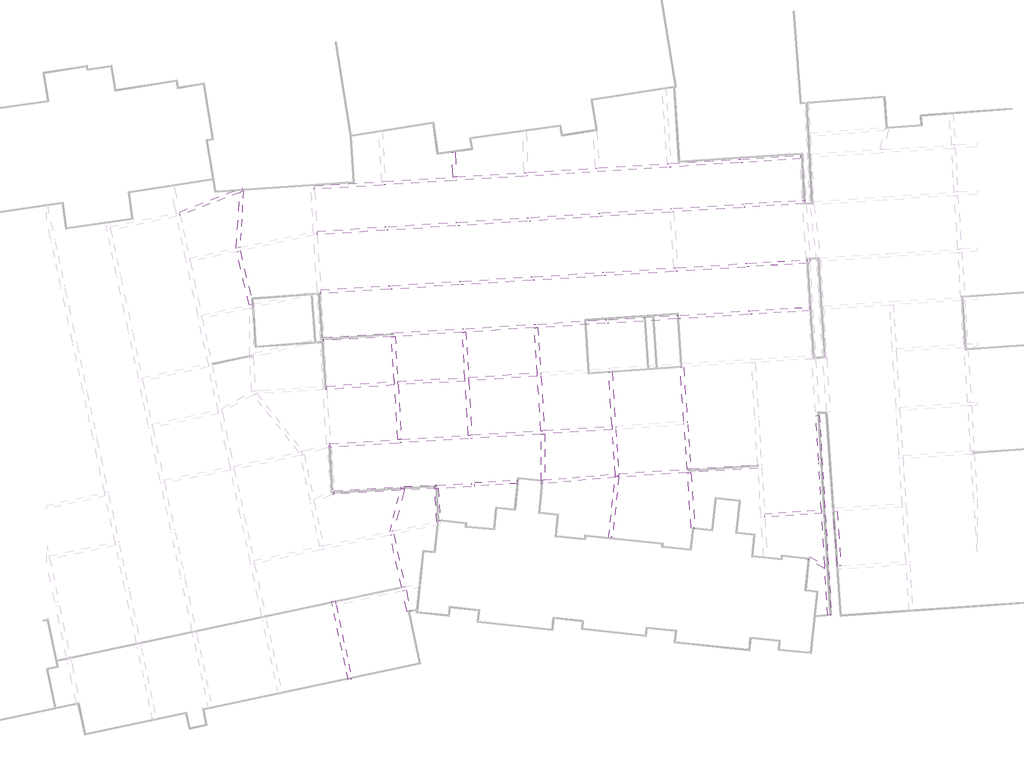
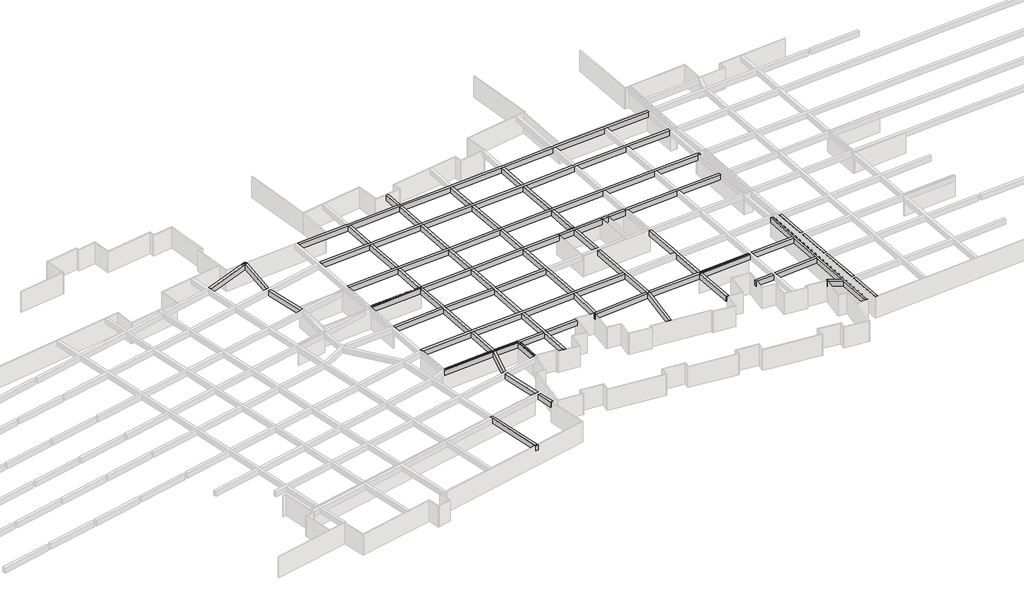
# One storey, part 11 of 14: 35 beams.
"""IFC4 building model written with IfcOpenShell, lengths in millimetres."""

import ifcopenshell
import ifcopenshell.guid

model = None  # the IFC model being written
_history = None  # IfcOwnerHistory: only IFC2X3 demands one
_inside = {}  # id of a spatial element -> (the spatial element, [elements in it])
_under = {}  # id of a project, library or spatial element -> (it, [spatial elements below it])
_declared = {}  # id of a project -> (the project, [libraries it declares])
_typed = {}  # id of a type object -> (the type object, [elements of that type])
_made_of = {}  # id of a material, layer set ... -> (it, [elements and type objects made of it])


def new_model(schema):
    """Start an empty IFC model of exactly this schema.

    Asked for "IFC4X3", IfcOpenShell would pick the latest addendum, in which some entities
    have other attributes; the version numbers below select the first issue.
    IFC2X3 requires an IfcOwnerHistory on every rooted entity: one is made here for all.
    """
    global model, _history
    if schema == "IFC4X3":
        model = ifcopenshell.file(schema_version=(4, 3, 0, 0))
    else:
        model = ifcopenshell.file(schema=schema)
    _inside.clear()
    _under.clear()
    _declared.clear()
    _typed.clear()
    _made_of.clear()
    _history = None
    if model.schema == "IFC2X3":
        org = make("IfcOrganization", Name="unknown")
        user = make(
            "IfcPersonAndOrganization",
            ThePerson=make("IfcPerson", FamilyName="unknown"),
            TheOrganization=org,
        )
        app = make(
            "IfcApplication",
            ApplicationDeveloper=org,
            Version="unknown",
            ApplicationFullName="unknown",
            ApplicationIdentifier="unknown",
        )
        _history = make(
            "IfcOwnerHistory",
            OwningUser=user,
            OwningApplication=app,
            ChangeAction="ADDED",
            CreationDate=0,
        )
    return model


def make(cls, **values):
    """One entity of the class cls with the attributes given. An attribute that is None is left unset."""
    return model.create_entity(
        cls, **{name: value for name, value in values.items() if value is not None}
    )


def rooted(cls, **values):
    """An entity with a GlobalId (a new one), such as an element, a storey or a relation."""
    return make(cls, GlobalId=ifcopenshell.guid.new(), OwnerHistory=_history, **values)


def si_unit(unit_type, name, prefix=None):
    """IfcSIUnit, for example si_unit("LENGTHUNIT", "METRE", prefix="MILLI")."""
    return make("IfcSIUnit", UnitType=unit_type, Prefix=prefix, Name=name)


def assignment(units):
    """IfcUnitAssignment: the units of a project."""
    return None if units is None else make("IfcUnitAssignment", Units=units)


def point(xyz):
    """IfcCartesianPoint."""
    return None if xyz is None else make("IfcCartesianPoint", Coordinates=xyz)


def direction(xyz):
    """IfcDirection."""
    return None if xyz is None else make("IfcDirection", DirectionRatios=xyz)


def frame(location, z_axis=None, x_axis=None):
    """IfcAxis2Placement3D, a coordinate frame: its origin and axes. An axis left out is left unset."""
    return make(
        "IfcAxis2Placement3D",
        Location=point(location),
        Axis=direction(z_axis),
        RefDirection=direction(x_axis),
    )


def origin():
    """The frame at (0, 0, 0) with its axes left unset."""
    return frame((0.0, 0.0, 0.0))


def place(relative_to, where):
    """IfcLocalPlacement: puts the frame where relative to a parent placement (None: the world)."""
    return make(
        "IfcLocalPlacement", PlacementRelTo=relative_to, RelativePlacement=where
    )


def context(
    kind, dimensions, precision=None, world=None, true_north=None, identifier=None
):
    """IfcGeometricRepresentationContext, for example the 3D "Model" context."""
    return make(
        "IfcGeometricRepresentationContext",
        ContextIdentifier=identifier,
        ContextType=kind,
        CoordinateSpaceDimension=dimensions,
        Precision=precision,
        WorldCoordinateSystem=world,
        TrueNorth=true_north,
    )


def project(units=None, contexts=None):
    """IfcProject with its units and contexts."""
    return rooted(
        "IfcProject",
        Name="project",
        RepresentationContexts=contexts,
        UnitsInContext=assignment(units),
    )


def spatial(cls, under=None, at=None, **own):
    """A site, building, storey or space (cls), placed at a placement, below another one or the project."""
    s = rooted(cls, ObjectPlacement=at, **own)
    if under is not None:
        _under.setdefault(under.id(), (under, []))[1].append(s)
    return s


def polyline(points):
    """IfcPolyline through the points."""
    return make("IfcPolyline", Points=[point(p) for p in points])


def outline(outer, holes=None, kind="AREA"):
    """IfcArbitraryClosedProfileDef: a profile drawn as a closed curve; with holes, ...WithVoids."""
    if holes is None:
        return make("IfcArbitraryClosedProfileDef", ProfileType=kind, OuterCurve=outer)
    return make(
        "IfcArbitraryProfileDefWithVoids",
        ProfileType=kind,
        OuterCurve=outer,
        InnerCurves=holes,
    )


def extrude(swept, where, along, depth):
    """IfcExtrudedAreaSolid: the profile swept, set in the frame where, extruded along a direction by depth."""
    return make(
        "IfcExtrudedAreaSolid",
        SweptArea=swept,
        Position=where,
        ExtrudedDirection=direction(along),
        Depth=depth,
    )


def faces_of(points, faces, orient=None, outer=None):
    """IfcFace entities. A face is a list of loops; a loop is a list of indices into points, from 0.

    orient and outer hold one flag for each loop. By default every Orientation is true, the
    first loop of a face is its IfcFaceOuterBound and the others are IfcFaceBound.
    """
    made = []
    for i, loops in enumerate(faces):
        bounds = []
        for j, loop in enumerate(loops):
            is_outer = j == 0 if outer is None else outer[i][j]
            bounds.append(
                make(
                    "IfcFaceOuterBound" if is_outer else "IfcFaceBound",
                    Bound=make("IfcPolyLoop", Polygon=[points[k] for k in loop]),
                    Orientation=True if orient is None else orient[i][j],
                )
            )
        made.append(make("IfcFace", Bounds=bounds))
    return made


def faceted_brep(points, faces, orient=None, outer=None, voids=None):
    """IfcFacetedBrep: a solid bounded by flat faces; with voids (closed shells), ...WithVoids."""
    shared = [point(p) for p in points]
    hull = make("IfcClosedShell", CfsFaces=faces_of(shared, faces, orient, outer))
    if voids is None:
        return make("IfcFacetedBrep", Outer=hull)
    return make(
        "IfcFacetedBrepWithVoids",
        Outer=hull,
        Voids=[
            make(cls, CfsFaces=faces_of(shared, fs, o, b)) for cls, fs, o, b in voids
        ],
    )


def shape(context_of_items, identifier, shape_type, items):
    """IfcShapeRepresentation: the items that make up one representation, for example the "Body"."""
    return make(
        "IfcShapeRepresentation",
        ContextOfItems=context_of_items,
        RepresentationIdentifier=identifier,
        RepresentationType=shape_type,
        Items=items,
    )


def made_of(thing, what):
    """Note that an element or type object is made of a material, layer set ...; save() writes the relation."""
    if what is not None:
        _made_of.setdefault(what.id(), (what, []))[1].append(thing)
    return thing


def element(
    cls,
    number,
    at=None,
    inside=None,
    cuts=None,
    type_object=None,
    material=None,
    context=None,
    identifier="Body",
    shape_type=None,
    held_by="IfcProductDefinitionShape",
    body=None,
    shapes=None,
    **own,
):
    """One element of the class cls, such as IfcWall. Its Tag is "e" and its number.

    at: its placement. inside: the storey or other place that contains it. cuts: it is an
    opening in that element (IfcRelVoidsElement). A single representation is given by context,
    identifier, shape_type and body (its items); several are given by shapes. held_by: the class
    of the entity that holds the representations. save() writes the other relations.
    """
    e = rooted(cls, Tag="e%d" % number, ObjectPlacement=at, **own)
    if body is not None:
        shapes = [shape(context, identifier, shape_type, body)]
    if shapes is not None:
        e.Representation = make(held_by, Representations=shapes)
    if inside is not None:
        _inside.setdefault(inside.id(), (inside, []))[1].append(e)
    if cuts is not None:
        rooted(
            "IfcRelVoidsElement", RelatingBuildingElement=cuts, RelatedOpeningElement=e
        )
    if type_object is not None:
        _typed.setdefault(type_object.id(), (type_object, []))[1].append(e)
    return made_of(e, material)


def aggregate(whole, parts):
    """IfcRelAggregates: a whole, such as a stair, and the parts it consists of."""
    return rooted("IfcRelAggregates", RelatingObject=whole, RelatedObjects=parts)


def save(model, path):
    """Write the relations noted so far, then the file.

    IfcRelAggregates (storeys below a building ...), IfcRelContainedInSpatialStructure (elements
    in a storey), IfcRelDefinesByType, IfcRelAssociatesMaterial and IfcRelDeclares: one each for
    every whole, place, type object, material and project.
    """
    for whole, parts in _under.values():
        aggregate(whole, parts)
    for where, things in _inside.values():
        rooted(
            "IfcRelContainedInSpatialStructure",
            RelatedElements=things,
            RelatingStructure=where,
        )
    for kind, things in _typed.values():
        rooted("IfcRelDefinesByType", RelatedObjects=things, RelatingType=kind)
    for what, things in _made_of.values():
        rooted("IfcRelAssociatesMaterial", RelatedObjects=things, RelatingMaterial=what)
    for by, libraries in _declared.values():
        rooted("IfcRelDeclares", RelatingContext=by, RelatedDefinitions=libraries)
    model.write(path)


model = new_model("IFC4")

# Units and contexts
model_context = context("Model", 3, world=origin())
ifc_project = project(units=[si_unit("LENGTHUNIT", "METRE", prefix="MILLI")], contexts=[model_context])

# Site, building, storey
site = spatial("IfcSite", under=ifc_project)
building = spatial("IfcBuilding", under=site)
storey = spatial("IfcBuildingStorey", under=building, Name="户型图", Elevation=0.0)

# Beams
placement = place(None, origin())
element("IfcBeam", 1, ObjectType="混凝土 - 矩形梁 : KL_beam", at=placement, inside=storey, context=model_context, shape_type="SweptSolid", body=[
    extrude(outline(polyline([(-202914.7402599, -137877.8870148), (-202523.4216199, -137794.7096702), (-201143.0968024, -143773.5533155), (-201534.4154425, -143856.7306602), (-202914.7402599, -137877.8870148)])), frame((0.0, 0.0, 2500.0), z_axis=(0.0, 0.0, 1.0), x_axis=(1.0, 0.0, 0.0)), (0.0, 0.0, 1.0), 800.0),
])
element("IfcBeam", 2, ObjectType="混凝土 - 矩形梁 : KL_beam", at=placement, inside=storey, context=model_context, shape_type="Brep", body=[
    faceted_brep([(-202198.6698141, -131106.9586968, 3300.0), (-202341.6322396, -130733.3790602, 3300.0), (-209337.422307, -133410.5461707, 3300.0), (-209253.2346635, -133806.6178935, 3300.0), (-202608.0467679, -131263.6201326, 3300.0), (-202198.6698141, -131106.9586968, 2500.0), (-209253.2346635, -133806.6178935, 2500.0), (-202608.0467679, -131263.6201326, 2500.0), (-202341.6322396, -130733.3790602, 2500.0), (-209337.422307, -133410.5461707, 2500.0)], [[[0, 1, 2, 3, 4]], [[5, 0, 4, 3, 6, 7]], [[8, 5, 7, 6, 9]], [[1, 8, 9, 2]], [[3, 2, 9, 6]], [[1, 0, 5, 8]]]),
])
element("IfcBeam", 3, ObjectType="混凝土 - 矩形梁 : KL_beam", at=placement, inside=storey, context=model_context, shape_type="SweptSolid", body=[
    extrude(outline(polyline([(-202608.0467679, -131263.6201326), (-202198.6698141, -131106.9586968), (-202549.7970747, -137391.3797083), (-202955.2359711, -137477.558406), (-202608.0467679, -131263.6201326)])), frame((0.0, 0.0, 2500.0), z_axis=(0.0, 0.0, 1.0), x_axis=(1.0, 0.0, 0.0)), (0.0, 0.0, 1.0), 800.0),
])
element("IfcBeam", 4, ObjectType="混凝土 - 矩形梁 : KL_beam", at=placement, inside=storey, context=model_context, shape_type="Brep", body=[
    faceted_brep([(-192560.4754291, -159419.8343743, 3300.0), (-192492.3575326, -159816.3897801, 3300.0), (-192314.4423096, -159805.402692, 3300.0), (-184837.7111202, -159343.679954, 3300.0), (-184438.4716687, -159319.0250709, 3300.0), (-176944.1403368, -158856.2154427, 3300.0), (-176544.8990965, -158831.5604492, 3300.0), (-168803.6666392, -158353.5035342, 3300.0), (-168403.6666392, -158328.8016839, 3300.0), (-160825.4800031, -157860.8136026, 3300.0), (-160851.087443, -157461.6329795, 3300.0), (-168417.1473431, -157928.8721787, 3300.0), (-168816.3897959, -157953.5272471, 3300.0), (-176568.3576498, -158432.2471224, 3300.0), (-176967.5988901, -158456.9021159, 3300.0), (-184463.1805596, -158919.7889583, 3300.0), (-184862.4200112, -158944.4438413, 3300.0), (-192451.8526704, -159413.1264165, 3300.0), (-192492.3575326, -159816.3897801, 2500.0), (-192314.4423096, -159805.402692, 2500.0), (-184837.7111202, -159343.679954, 2500.0), (-184438.4716687, -159319.0250709, 2500.0), (-176944.1403368, -158856.2154427, 2500.0), (-176544.8990965, -158831.5604492, 2500.0), (-168803.6666392, -158353.5035342, 2500.0), (-168403.6666392, -158328.8016839, 2500.0), (-160825.4800031, -157860.8136026, 2500.0), (-192560.4754291, -159419.8343743, 2500.0), (-192451.8526704, -159413.1264165, 2500.0), (-184862.4200112, -158944.4438413, 2500.0), (-184463.1805596, -158919.7889583, 2500.0), (-176967.5988901, -158456.9021159, 2500.0), (-176568.3576498, -158432.2471224, 2500.0), (-168816.3897959, -157953.5272471, 2500.0), (-168417.1473431, -157928.8721787, 2500.0), (-160851.087443, -157461.6329795, 2500.0)], [[[0, 1, 2, 3, 4, 5, 6, 7, 8, 9, 10, 11, 12, 13, 14, 15, 16, 17]], [[1, 18, 19, 20, 21, 22, 23, 24, 25, 26, 9, 8, 7, 6, 5, 4, 3, 2]], [[18, 27, 28, 29, 30, 31, 32, 33, 34, 35, 26, 25, 24, 23, 22, 21, 20, 19]], [[27, 0, 17, 16, 15, 14, 13, 12, 11, 10, 35, 34, 33, 32, 31, 30, 29, 28]], [[0, 27, 18, 1]], [[10, 9, 26, 35]]]),
])
element("IfcBeam", 5, ObjectType="混凝土 - 矩形梁 : KL_beam", at=placement, inside=storey, context=model_context, shape_type="SweptSolid", body=[
    extrude(outline(polyline([(-192825.7838606, -153358.014199), (-192850.4395595, -152958.7615342), (-185265.7016346, -152428.3849916), (-185240.9919528, -152827.6338816), (-192825.7838606, -153358.014199)])), frame((0.0, 0.0, 2500.0), z_axis=(0.0, 0.0, 1.0), x_axis=(1.0, 0.0, 0.0)), (0.0, 0.0, 1.0), 800.0),
])
element("IfcBeam", 6, ObjectType="混凝土 - 矩形梁 : KL_beam", at=placement, inside=storey, context=model_context, shape_type="SweptSolid", body=[
    extrude(outline(polyline([(-184841.8420261, -152801.5324931), (-184866.5520206, -152402.2785506), (-177346.4442733, -152008.1664036), (-177322.9853569, -152407.4859123), (-184841.8420261, -152801.5324931)])), frame((0.0, 0.0, 2500.0), z_axis=(0.0, 0.0, 1.0), x_axis=(1.0, 0.0, 0.0)), (0.0, 0.0, 1.0), 800.0),
])
element("IfcBeam", 7, ObjectType="混凝土 - 矩形梁 : KL_beam", at=placement, inside=storey, context=model_context, shape_type="SweptSolid", body=[
    extrude(outline(polyline([(-176923.5589701, -152385.982497), (-176947.018872, -151986.646214), (-169243.4812831, -151447.9623897), (-169217.2773821, -151847.1067937), (-176923.5589701, -152385.982497)])), frame((0.0, 0.0, 2500.0), z_axis=(0.0, 0.0, 1.0), x_axis=(1.0, 0.0, 0.0)), (0.0, 0.0, 1.0), 800.0),
])
element("IfcBeam", 8, ObjectType="混凝土 - 矩形梁 : KL_beam", at=placement, inside=storey, context=model_context, shape_type="Brep", body=[
    faceted_brep([(-193187.2993167, -147503.9514384, 3300.0), (-193162.6444274, -147903.1909921, 3300.0), (-185575.1107179, -147429.0800922, 3300.0), (-185175.8892562, -147404.1345362, 3300.0), (-177644.564777, -146933.5358987, 3300.0), (-177245.3406164, -146908.5901741, 3300.0), (-169572.9653748, -146429.1779079, 3300.0), (-169173.7420004, -146404.2322325, 3300.0), (-161590.815531, -145930.4092183, 3300.0), (-161191.5935908, -145905.4636325, 3300.0), (-153570.081579, -145429.2295811, 3300.0), (-153170.8601875, -145404.2840296, 3300.0), (-145554.3512097, -144928.3625953, 3300.0), (-145155.1298182, -144903.4170437, 3300.0), (-138723.9209548, -144501.5596895, 3300.0), (-138748.8665064, -144102.338298, 3300.0), (-145180.0753697, -144504.1956522, 3300.0), (-145579.2967612, -144529.1412037, 3300.0), (-153195.805739, -145005.062638, 3300.0), (-153595.0271306, -145030.0081896, 3300.0), (-161217.200993, -145506.283597, 3300.0), (-161616.4229331, -145531.2291828, 3300.0), (-169199.9457941, -146005.0894629, 3300.0), (-169599.1691684, -146030.0351383, 3300.0), (-177268.799227, -146509.2758703, 3300.0), (-177668.0233877, -146534.2215949, 3300.0), (-185200.5981513, -147004.8983571, 3300.0), (-185599.819613, -147029.843913, 3300.0), (-193162.6444274, -147903.1909921, 2500.0), (-185575.1107179, -147429.0800922, 2500.0), (-185175.8892562, -147404.1345362, 2500.0), (-177644.564777, -146933.5358987, 2500.0), (-177245.3406164, -146908.5901741, 2500.0), (-169572.9653748, -146429.1779079, 2500.0), (-169173.7420004, -146404.2322325, 2500.0), (-161590.815531, -145930.4092183, 2500.0), (-161191.5935908, -145905.4636325, 2500.0), (-153570.081579, -145429.2295811, 2500.0), (-153170.8601875, -145404.2840296, 2500.0), (-145554.3512097, -144928.3625953, 2500.0), (-145155.1298182, -144903.4170437, 2500.0), (-138723.9209548, -144501.5596895, 2500.0), (-193187.2993167, -147503.9514384, 2500.0), (-185599.819613, -147029.843913, 2500.0), (-185200.5981513, -147004.8983571, 2500.0), (-177668.0233877, -146534.2215949, 2500.0), (-177268.799227, -146509.2758703, 2500.0), (-169599.1691684, -146030.0351383, 2500.0), (-169199.9457941, -146005.0894629, 2500.0), (-161616.4229331, -145531.2291828, 2500.0), (-161217.200993, -145506.283597, 2500.0), (-153595.0271306, -145030.0081896, 2500.0), (-153195.805739, -145005.062638, 2500.0), (-145579.2967612, -144529.1412037, 2500.0), (-145180.0753697, -144504.1956522, 2500.0), (-138748.8665064, -144102.338298, 2500.0)], [[[0, 1, 2, 3, 4, 5, 6, 7, 8, 9, 10, 11, 12, 13, 14, 15, 16, 17, 18, 19, 20, 21, 22, 23, 24, 25, 26, 27]], [[1, 28, 29, 30, 31, 32, 33, 34, 35, 36, 37, 38, 39, 40, 41, 14, 13, 12, 11, 10, 9, 8, 7, 6, 5, 4, 3, 2]], [[28, 42, 43, 44, 45, 46, 47, 48, 49, 50, 51, 52, 53, 54, 55, 41, 40, 39, 38, 37, 36, 35, 34, 33, 32, 31, 30, 29]], [[42, 0, 27, 26, 25, 24, 23, 22, 21, 20, 19, 18, 17, 16, 15, 55, 54, 53, 52, 51, 50, 49, 48, 47, 46, 45, 44, 43]], [[1, 0, 42, 28]], [[15, 14, 41, 55]]]),
])
element("IfcBeam", 9, ObjectType="混凝土 - 矩形梁 : KL_beam", at=placement, inside=storey, context=model_context, shape_type="Brep", body=[
    faceted_brep([(-138657.072748, -139157.4098254, 3300.0), (-138682.0182996, -138758.1884339, 3300.0), (-139081.2396911, -138783.1339854, 3300.0), (-145512.4485544, -139184.9913397, 3300.0), (-145911.669946, -139209.9368912, 3300.0), (-153528.1789238, -139685.8583255, 3300.0), (-153927.4003153, -139710.803877, 3300.0), (-161558.3926399, -140187.6303106, 3300.0), (-161957.61458, -140212.5758964, 3300.0), (-169549.0837289, -140686.9327042, 3300.0), (-169948.3071033, -140711.8783797, 3300.0), (-177581.3604919, -141188.8335999, 3300.0), (-177980.5846526, -141213.7793244, 3300.0), (-185529.8181381, -141685.4970154, 3300.0), (-185929.0395998, -141710.4425713, 3300.0), (-193515.7997336, -142184.505134, 3300.0), (-193491.1448443, -142583.7446877, 3300.0), (-185904.3307047, -142109.6787505, 3300.0), (-185505.109243, -142084.7331945, 3300.0), (-177957.1260419, -141613.0936282, 3300.0), (-177557.9018812, -141588.1479037, 3300.0), (-169922.1033096, -141111.0211493, 3300.0), (-169522.8799353, -141086.0754739, 3300.0), (-161932.0071779, -140611.7559319, 3300.0), (-161532.7852377, -140586.810346, 3300.0), (-153902.4547638, -140110.0252686, 3300.0), (-153503.2333722, -140085.079717, 3300.0), (-145886.7243944, -139609.1582827, 3300.0), (-145487.5030029, -139584.2127312, 3300.0), (-139056.2941396, -139182.355377, 3300.0), (-138657.072748, -139157.4098254, 2500.0), (-193491.1448443, -142583.7446877, 2500.0), (-185904.3307047, -142109.6787505, 2500.0), (-185505.109243, -142084.7331945, 2500.0), (-177957.1260419, -141613.0936282, 2500.0), (-177557.9018812, -141588.1479037, 2500.0), (-169922.1033096, -141111.0211493, 2500.0), (-169522.8799353, -141086.0754739, 2500.0), (-161932.0071779, -140611.7559319, 2500.0), (-161532.7852377, -140586.810346, 2500.0), (-153902.4547638, -140110.0252686, 2500.0), (-153503.2333722, -140085.079717, 2500.0), (-145886.7243944, -139609.1582827, 2500.0), (-145487.5030029, -139584.2127312, 2500.0), (-139056.2941396, -139182.355377, 2500.0), (-138682.0182996, -138758.1884339, 2500.0), (-193515.7997336, -142184.505134, 2500.0), (-185929.0395998, -141710.4425713, 2500.0), (-185529.8181381, -141685.4970154, 2500.0), (-177980.5846526, -141213.7793244, 2500.0), (-177581.3604919, -141188.8335999, 2500.0), (-169948.3071033, -140711.8783797, 2500.0), (-169549.0837289, -140686.9327042, 2500.0), (-161957.61458, -140212.5758964, 2500.0), (-161558.3926399, -140187.6303106, 2500.0), (-153927.4003153, -139710.803877, 2500.0), (-153528.1789238, -139685.8583255, 2500.0), (-145911.669946, -139209.9368912, 2500.0), (-145512.4485544, -139184.9913397, 2500.0), (-139081.2396911, -138783.1339854, 2500.0)], [[[0, 1, 2, 3, 4, 5, 6, 7, 8, 9, 10, 11, 12, 13, 14, 15, 16, 17, 18, 19, 20, 21, 22, 23, 24, 25, 26, 27, 28, 29]], [[30, 0, 29, 28, 27, 26, 25, 24, 23, 22, 21, 20, 19, 18, 17, 16, 31, 32, 33, 34, 35, 36, 37, 38, 39, 40, 41, 42, 43, 44]], [[45, 30, 44, 43, 42, 41, 40, 39, 38, 37, 36, 35, 34, 33, 32, 31, 46, 47, 48, 49, 50, 51, 52, 53, 54, 55, 56, 57, 58, 59]], [[1, 45, 59, 58, 57, 56, 55, 54, 53, 52, 51, 50, 49, 48, 47, 46, 15, 14, 13, 12, 11, 10, 9, 8, 7, 6, 5, 4, 3, 2]], [[16, 15, 46, 31]], [[1, 0, 30, 45]]]),
])
element("IfcBeam", 10, ObjectType="混凝土 - 矩形梁 : KL_beam", at=placement, inside=storey, context=model_context, shape_type="Brep", body=[
    faceted_brep([(-139297.110977, -132093.4842358, 3300.0), (-139271.5629231, -132492.6675232, 3300.0), (-139271.5629231, -132492.6675232, 2500.0), (-139297.110977, -132093.4842358, 2500.0), (-139498.4407131, -132106.369502, 3300.0), (-145929.0430666, -132517.9332638, 3300.0), (-146328.2268086, -132543.4813468, 3300.0), (-153944.0174942, -133030.8981222, 3300.0), (-154343.2012363, -133056.4462052, 3300.0), (-161984.4856938, -133545.4946027, 3300.0), (-162383.6689856, -133571.0426569, 3300.0), (-169984.3078382, -134057.4897027, 3300.0), (-170383.4916641, -134083.0377911, 3300.0), (-177970.2809924, -134568.5984562, 3300.0), (-178369.4697473, -134594.14686, 3300.0), (-185938.7226909, -135078.5851822, 3300.0), (-186337.9068602, -135104.1332925, 3300.0), (-193923.0662732, -135589.5896417, 3300.0), (-193898.4113287, -135988.8300888, 3300.0), (-186313.1979149, -135503.3702836, 3300.0), (-185914.0137455, -135477.8221732, 3300.0), (-178346.010978, -134993.4638633, 3300.0), (-177946.8222231, -134967.9154595, 3300.0), (-170357.2879652, -134482.1791167, 3300.0), (-169958.1041394, -134456.6310283, 3300.0), (-162358.0616183, -133970.2221482, 3300.0), (-161958.8783265, -133944.674094, 3300.0), (-154318.2556563, -133455.6680514, 3300.0), (-153919.0719143, -133430.1199684, 3300.0), (-146303.2812287, -132942.703193, 3300.0), (-145904.0974866, -132917.15511, 3300.0), (-139473.4951331, -132505.5913482, 3300.0), (-193898.4113287, -135988.8300888, 2500.0), (-186313.1979149, -135503.3702836, 2500.0), (-185914.0137455, -135477.8221732, 2500.0), (-178346.010978, -134993.4638633, 2500.0), (-177946.8222231, -134967.9154595, 2500.0), (-170357.2879652, -134482.1791167, 2500.0), (-169958.1041394, -134456.6310283, 2500.0), (-162358.0616183, -133970.2221482, 2500.0), (-161958.8783265, -133944.674094, 2500.0), (-154318.2556563, -133455.6680514, 2500.0), (-153919.0719143, -133430.1199684, 2500.0), (-146303.2812287, -132942.703193, 2500.0), (-145904.0974866, -132917.15511, 2500.0), (-139473.4951331, -132505.5913482, 2500.0), (-193923.0662732, -135589.5896417, 2500.0), (-186337.9068602, -135104.1332925, 2500.0), (-185938.7226909, -135078.5851822, 2500.0), (-178369.4697473, -134594.14686, 2500.0), (-177970.2809924, -134568.5984562, 2500.0), (-170383.4916641, -134083.0377911, 2500.0), (-169984.3078382, -134057.4897027, 2500.0), (-162383.6689856, -133571.0426569, 2500.0), (-161984.4856938, -133545.4946027, 2500.0), (-154343.2012363, -133056.4462052, 2500.0), (-153944.0174942, -133030.8981222, 2500.0), (-146328.2268086, -132543.4813468, 2500.0), (-145929.0430666, -132517.9332638, 2500.0), (-139498.4407131, -132106.369502, 2500.0)], [[[0, 1, 2, 3]], [[1, 0, 4, 5, 6, 7, 8, 9, 10, 11, 12, 13, 14, 15, 16, 17, 18, 19, 20, 21, 22, 23, 24, 25, 26, 27, 28, 29, 30, 31]], [[2, 1, 31, 30, 29, 28, 27, 26, 25, 24, 23, 22, 21, 20, 19, 18, 32, 33, 34, 35, 36, 37, 38, 39, 40, 41, 42, 43, 44, 45]], [[3, 2, 45, 44, 43, 42, 41, 40, 39, 38, 37, 36, 35, 34, 33, 32, 46, 47, 48, 49, 50, 51, 52, 53, 54, 55, 56, 57, 58, 59]], [[0, 3, 59, 58, 57, 56, 55, 54, 53, 52, 51, 50, 49, 48, 47, 46, 17, 16, 15, 14, 13, 12, 11, 10, 9, 8, 7, 6, 5, 4]], [[18, 17, 46, 32]]]),
])
element("IfcBeam", 11, ObjectType="混凝土 - 矩形梁 : KL_beam", at=placement, inside=storey, context=model_context, shape_type="Brep", body=[
    faceted_brep([(-139743.8905829, -127093.4326594, 3300.0), (-139718.9450314, -127492.6540509, 3300.0), (-139718.9450314, -127492.6540509, 2500.0), (-139743.8905829, -127093.4326594, 2500.0), (-139811.4129822, -127097.6518308, 3300.0), (-146242.6218456, -127499.509185, 3300.0), (-146641.8432371, -127524.4547366, 3300.0), (-154286.932885, -128002.1620485, 3300.0), (-154686.1542765, -128027.1076001, 3300.0), (-162299.8992046, -128502.8563213, 3300.0), (-162699.1205962, -128527.8018729, 3300.0), (-170294.3543471, -129002.3939138, 3300.0), (-170693.7267176, -129027.3488993, 3300.0), (-178268.754866, -129500.6783829, 3300.0), (-178667.9762575, -129525.6239344, 3300.0), (-186253.1826967, -129999.5894137, 3300.0), (-186652.4040882, -130024.5349652, 3300.0), (-194237.4651433, -130498.49136, 3300.0), (-194212.810254, -130897.7309138, 3300.0), (-186627.5769, -130423.7637527, 3300.0), (-186228.3554383, -130398.8181968, 3300.0), (-178643.775561, -129924.8918686, 3300.0), (-178244.5514003, -129899.946144, 3300.0), (-170689.1062046, -129427.8403112, 3300.0), (-170289.8828302, -129402.8946358, 3300.0), (-154632.6280549, -128424.5431139, 3300.0), (-154233.4066634, -128399.5975624, 3300.0), (-146616.8976856, -127923.6761281, 3300.0), (-146217.676294, -127898.7305766, 3300.0), (-139786.4674307, -127496.8732223, 3300.0), (-194212.810254, -130897.7309138, 2500.0), (-186627.5769, -130423.7637527, 2500.0), (-186228.3554383, -130398.8181968, 2500.0), (-178643.775561, -129924.8918686, 2500.0), (-178244.5514003, -129899.946144, 2500.0), (-170689.1062046, -129427.8403112, 2500.0), (-170289.8828302, -129402.8946358, 2500.0), (-154632.6280549, -128424.5431139, 2500.0), (-154233.4066634, -128399.5975624, 2500.0), (-146616.8976856, -127923.6761281, 2500.0), (-146217.676294, -127898.7305766, 2500.0), (-139786.4674307, -127496.8732223, 2500.0), (-194237.4651433, -130498.49136, 2500.0), (-186652.4040882, -130024.5349652, 2500.0), (-186253.1826967, -129999.5894137, 2500.0), (-178667.9762575, -129525.6239344, 2500.0), (-178268.754866, -129500.6783829, 2500.0), (-170693.7267176, -129027.3488993, 2500.0), (-170294.3543471, -129002.3939138, 2500.0), (-162699.1205962, -128527.8018729, 2500.0), (-162299.8992046, -128502.8563213, 2500.0), (-154686.1542765, -128027.1076001, 2500.0), (-154286.932885, -128002.1620485, 2500.0), (-146641.8432371, -127524.4547366, 2500.0), (-146242.6218456, -127499.509185, 2500.0), (-139811.4129822, -127097.6518308, 2500.0)], [[[0, 1, 2, 3]], [[1, 0, 4, 5, 6, 7, 8, 9, 10, 11, 12, 13, 14, 15, 16, 17, 18, 19, 20, 21, 22, 23, 24, 25, 26, 27, 28, 29]], [[2, 1, 29, 28, 27, 26, 25, 24, 23, 22, 21, 20, 19, 18, 30, 31, 32, 33, 34, 35, 36, 37, 38, 39, 40, 41]], [[3, 2, 41, 40, 39, 38, 37, 36, 35, 34, 33, 32, 31, 30, 42, 43, 44, 45, 46, 47, 48, 49, 50, 51, 52, 53, 54, 55]], [[0, 3, 55, 54, 53, 52, 51, 50, 49, 48, 47, 46, 45, 44, 43, 42, 17, 16, 15, 14, 13, 12, 11, 10, 9, 8, 7, 6, 5, 4]], [[18, 17, 42, 30]]]),
])
element("IfcBeam", 12, ObjectType="混凝土 - 矩形梁 : KL_beam", at=placement, inside=storey, context=model_context, shape_type="SweptSolid", body=[
    extrude(outline(polyline([(-178841.5502041, -126747.7966985), (-178442.3288125, -126722.8511469), (-178268.754866, -129500.6783829), (-178667.9762575, -129525.6239344), (-178841.5502041, -126747.7966985)])), frame((0.0, 0.0, 2500.0), z_axis=(0.0, 0.0, 1.0), x_axis=(1.0, 0.0, 0.0)), (0.0, 0.0, 1.0), 800.0),
])
element("IfcBeam", 13, ObjectType="混凝土 - 矩形梁 : KL_beam", at=placement, inside=storey, context=model_context, shape_type="Brep", body=[
    faceted_brep([(-184121.5948071, -164438.9912635, 3300.0), (-184135.7391466, -164210.4528361, 3300.0), (-184438.4716687, -159319.0250709, 3300.0), (-184837.7111202, -159343.679954, 3300.0), (-184535.0914777, -164233.283857, 3300.0), (-184524.6431485, -164402.1036687, 3300.0), (-184837.7111202, -159343.679954, 2500.0), (-184535.0914777, -164233.283857, 2500.0), (-184524.6431485, -164402.1036687, 2500.0), (-184438.4716687, -159319.0250709, 2500.0), (-184135.7391466, -164210.4528361, 2500.0), (-184121.5948071, -164438.9912635, 2500.0)], [[[0, 1, 2, 3, 4, 5]], [[5, 4, 3, 6, 7, 8]], [[8, 7, 6, 9, 10, 11]], [[2, 1, 0, 11, 10, 9]], [[3, 2, 9, 6]], [[0, 5, 8, 11]]]),
    faceted_brep([(-186627.5769, -130423.7637527, 3300.0), (-186228.3554383, -130398.8181968, 3300.0), (-186228.3554383, -130398.8181968, 2500.0), (-186627.5769, -130423.7637527, 2500.0), (-185938.7226909, -135078.5851822, 3300.0), (-186337.9068602, -135104.1332925, 3300.0), (-186337.9068602, -135104.1332925, 2500.0), (-185938.7226909, -135078.5851822, 2500.0)], [[[0, 1, 2, 3]], [[4, 5, 6, 7]], [[1, 0, 5, 4]], [[0, 3, 6, 5]], [[3, 2, 7, 6]], [[2, 1, 4, 7]]]),
    faceted_brep([(-184463.1805596, -158919.7889583, 3300.0), (-184862.4200112, -158944.4438413, 3300.0), (-184862.4200112, -158944.4438413, 2500.0), (-184463.1805596, -158919.7889583, 2500.0), (-184841.8420261, -152801.5324931, 3300.0), (-184866.5520206, -152402.2785506, 3300.0), (-185175.8892562, -147404.1345362, 3300.0), (-185575.1107179, -147429.0800922, 3300.0), (-185265.7016346, -152428.3849916, 3300.0), (-185240.9919528, -152827.6338816, 3300.0), (-185575.1107179, -147429.0800922, 2500.0), (-185265.7016346, -152428.3849916, 2500.0), (-185240.9919528, -152827.6338816, 2500.0), (-185175.8892562, -147404.1345362, 2500.0), (-184866.5520206, -152402.2785506, 2500.0), (-184841.8420261, -152801.5324931, 2500.0)], [[[0, 1, 2, 3]], [[1, 0, 4, 5, 6, 7, 8, 9]], [[2, 1, 9, 8, 7, 10, 11, 12]], [[3, 2, 12, 11, 10, 13, 14, 15]], [[0, 3, 15, 14, 13, 6, 5, 4]], [[7, 6, 13, 10]]]),
    faceted_brep([(-185200.5981513, -147004.8983571, 3300.0), (-185599.819613, -147029.843913, 3300.0), (-185599.819613, -147029.843913, 2500.0), (-185200.5981513, -147004.8983571, 2500.0), (-185505.109243, -142084.7331945, 3300.0), (-185904.3307047, -142109.6787505, 3300.0), (-185904.3307047, -142109.6787505, 2500.0), (-185505.109243, -142084.7331945, 2500.0)], [[[0, 1, 2, 3]], [[1, 0, 4, 5]], [[2, 1, 5, 6]], [[3, 2, 6, 7]], [[0, 3, 7, 4]], [[5, 4, 7, 6]]]),
    faceted_brep([(-185529.8181381, -141685.4970154, 3300.0), (-185929.0395998, -141710.4425713, 3300.0), (-185929.0395998, -141710.4425713, 2500.0), (-185529.8181381, -141685.4970154, 2500.0), (-185914.0137455, -135477.8221732, 3300.0), (-186313.1979149, -135503.3702836, 3300.0), (-186313.1979149, -135503.3702836, 2500.0), (-185914.0137455, -135477.8221732, 2500.0)], [[[0, 1, 2, 3]], [[1, 0, 4, 5]], [[2, 1, 5, 6]], [[3, 2, 6, 7]], [[0, 3, 7, 4]], [[5, 4, 7, 6]]]),
])
element("IfcBeam", 14, ObjectType="混凝土 - 矩形梁 : KL_beam", at=placement, inside=storey, context=model_context, shape_type="Brep", body=[
    faceted_brep([(-175959.7601738, -168791.8409064, 3300.0), (-176359.0717079, -168815.2993544, 3300.0), (-176359.0717079, -168815.2993544, 2500.0), (-175959.7601738, -168791.8409064, 2500.0), (-176231.8313354, -164160.6243376, 3300.0), (-176255.2897834, -163761.3128036, 3300.0), (-176544.8990965, -158831.5604492, 3300.0), (-176944.1403368, -158856.2154427, 3300.0), (-176651.7057707, -163834.0594731, 3300.0), (-176628.2473228, -164233.3710071, 3300.0), (-176944.1403368, -158856.2154427, 2500.0), (-176651.7057707, -163834.0594731, 2500.0), (-176628.2473228, -164233.3710071, 2500.0), (-176544.8990965, -158831.5604492, 2500.0), (-176255.2897834, -163761.3128036, 2500.0), (-176231.8313354, -164160.6243376, 2500.0)], [[[0, 1, 2, 3]], [[1, 0, 4, 5, 6, 7, 8, 9]], [[2, 1, 9, 8, 7, 10, 11, 12]], [[3, 2, 12, 11, 10, 13, 14, 15]], [[0, 3, 15, 14, 13, 6, 5, 4]], [[7, 6, 13, 10]]]),
    faceted_brep([(-178643.775561, -129924.8918686, 3300.0), (-178244.5514003, -129899.946144, 3300.0), (-178244.5514003, -129899.946144, 2500.0), (-178643.775561, -129924.8918686, 2500.0), (-177970.2809924, -134568.5984562, 3300.0), (-178369.4697473, -134594.14686, 3300.0), (-178369.4697473, -134594.14686, 2500.0), (-177970.2809924, -134568.5984562, 2500.0)], [[[0, 1, 2, 3]], [[4, 5, 6, 7]], [[1, 0, 5, 4]], [[0, 3, 6, 5]], [[3, 2, 7, 6]], [[2, 1, 4, 7]]]),
    faceted_brep([(-176568.3576498, -158432.2471224, 3300.0), (-176967.5988901, -158456.9021159, 3300.0), (-176967.5988901, -158456.9021159, 2500.0), (-176568.3576498, -158432.2471224, 2500.0), (-176923.5589701, -152385.982497, 3300.0), (-176947.018872, -151986.646214, 3300.0), (-177245.3406164, -146908.5901741, 3300.0), (-177644.564777, -146933.5358987, 3300.0), (-177346.4442733, -152008.1664036, 3300.0), (-177322.9853569, -152407.4859123, 3300.0), (-177644.564777, -146933.5358987, 2500.0), (-177346.4442733, -152008.1664036, 2500.0), (-177322.9853569, -152407.4859123, 2500.0), (-177245.3406164, -146908.5901741, 2500.0), (-176947.018872, -151986.646214, 2500.0), (-176923.5589701, -152385.982497, 2500.0)], [[[0, 1, 2, 3]], [[1, 0, 4, 5, 6, 7, 8, 9]], [[2, 1, 9, 8, 7, 10, 11, 12]], [[3, 2, 12, 11, 10, 13, 14, 15]], [[0, 3, 15, 14, 13, 6, 5, 4]], [[7, 6, 13, 10]]]),
    faceted_brep([(-177268.799227, -146509.2758703, 3300.0), (-177668.0233877, -146534.2215949, 3300.0), (-177668.0233877, -146534.2215949, 2500.0), (-177268.799227, -146509.2758703, 2500.0), (-177557.9018812, -141588.1479037, 3300.0), (-177957.1260419, -141613.0936282, 3300.0), (-177957.1260419, -141613.0936282, 2500.0), (-177557.9018812, -141588.1479037, 2500.0)], [[[0, 1, 2, 3]], [[1, 0, 4, 5]], [[2, 1, 5, 6]], [[3, 2, 6, 7]], [[0, 3, 7, 4]], [[5, 4, 7, 6]]]),
    faceted_brep([(-177581.3604919, -141188.8335999, 3300.0), (-177980.5846526, -141213.7793244, 3300.0), (-177980.5846526, -141213.7793244, 2500.0), (-177581.3604919, -141188.8335999, 2500.0), (-177946.8222231, -134967.9154595, 3300.0), (-178346.010978, -134993.4638633, 3300.0), (-178346.010978, -134993.4638633, 2500.0), (-177946.8222231, -134967.9154595, 2500.0)], [[[0, 1, 2, 3]], [[1, 0, 4, 5]], [[2, 1, 5, 6]], [[3, 2, 6, 7]], [[0, 3, 7, 4]], [[5, 4, 7, 6]]]),
])
element("IfcBeam", 15, ObjectType="混凝土 - 矩形梁 : KL_beam", at=placement, inside=storey, context=model_context, shape_type="Brep", body=[
    faceted_brep([(-170289.8828302, -129402.8946358, 3300.0), (-170689.1062046, -129427.8403112, 3300.0), (-170383.4916641, -134083.0377911, 3300.0), (-169984.3078382, -134057.4897027, 3300.0), (-170289.8828302, -129402.8946358, 2500.0), (-169984.3078382, -134057.4897027, 2500.0), (-170689.1062046, -129427.8403112, 2500.0), (-170383.4916641, -134083.0377911, 2500.0)], [[[0, 1, 2, 3]], [[4, 0, 3, 5]], [[6, 4, 5, 7]], [[1, 6, 7, 2]], [[1, 0, 4, 6]], [[3, 2, 7, 5]]]),
    faceted_brep([(-168417.1473431, -157928.8721787, 3300.0), (-168816.3897959, -157953.5272471, 3300.0), (-168816.3897959, -157953.5272471, 2500.0), (-168417.1473431, -157928.8721787, 2500.0), (-169572.9653748, -146429.1779079, 3300.0), (-169173.7420004, -146404.2322325, 3300.0), (-169173.7420004, -146404.2322325, 2500.0), (-169572.9653748, -146429.1779079, 2500.0), (-168818.123542, -151821.1019553, 3300.0), (-168844.3273357, -151421.9591856, 3300.0), (-169243.4812831, -151447.9623897, 3300.0), (-169217.2773821, -151847.1067937, 3300.0), (-168818.123542, -151821.1019553, 2500.0), (-168844.3273357, -151421.9591856, 2500.0), (-169217.2773821, -151847.1067937, 2500.0), (-169243.4812831, -151447.9623897, 2500.0)], [[[0, 1, 2, 3]], [[4, 5, 6, 7]], [[1, 0, 8, 9, 5, 4, 10, 11]], [[0, 3, 12, 13, 6, 5, 9, 8]], [[3, 2, 14, 15, 7, 6, 13, 12]], [[2, 1, 11, 10, 4, 7, 15, 14]]]),
    faceted_brep([(-169199.9457941, -146005.0894629, 3300.0), (-169599.1691684, -146030.0351383, 3300.0), (-169599.1691684, -146030.0351383, 2500.0), (-169199.9457941, -146005.0894629, 2500.0), (-169922.1033096, -141111.0211493, 3300.0), (-169522.8799353, -141086.0754739, 3300.0), (-169522.8799353, -141086.0754739, 2500.0), (-169922.1033096, -141111.0211493, 2500.0)], [[[0, 1, 2, 3]], [[4, 5, 6, 7]], [[1, 0, 5, 4]], [[0, 3, 6, 5]], [[3, 2, 7, 6]], [[2, 1, 4, 7]]]),
    faceted_brep([(-169549.0837289, -140686.9327042, 3300.0), (-169948.3071033, -140711.8783797, 3300.0), (-169948.3071033, -140711.8783797, 2500.0), (-169549.0837289, -140686.9327042, 2500.0), (-170357.2879652, -134482.1791167, 3300.0), (-169958.1041394, -134456.6310283, 3300.0), (-169958.1041394, -134456.6310283, 2500.0), (-170357.2879652, -134482.1791167, 2500.0)], [[[0, 1, 2, 3]], [[4, 5, 6, 7]], [[1, 0, 5, 4]], [[0, 3, 6, 5]], [[3, 2, 7, 6]], [[2, 1, 4, 7]]]),
])
element("IfcBeam", 16, ObjectType="混凝土 - 矩形梁 : KL_beam", at=placement, inside=storey, context=model_context, shape_type="Brep", body=[
    faceted_brep([(-162282.0891274, -128906.3145557, 3300.0), (-162282.0891274, -128906.3145557, 2500.0), (-162681.2686143, -128931.9219227, 2500.0), (-162681.2686143, -128931.9219227, 3300.0), (-161984.4856938, -133545.4946027, 3300.0), (-162383.6689856, -133571.0426569, 3300.0), (-162383.6689856, -133571.0426569, 2500.0), (-161984.4856938, -133545.4946027, 2500.0)], [[[0, 1, 2, 3]], [[4, 5, 6, 7]], [[0, 3, 5, 4]], [[3, 2, 6, 5]], [[2, 1, 7, 6]], [[1, 0, 4, 7]]]),
    faceted_brep([(-160091.5761626, -163053.0443613, 3300.0), (-160110.1828128, -162762.9952879, 3300.0), (-160426.3434263, -157834.5373332, 3300.0), (-160451.9512168, -157435.3512451, 3300.0), (-160844.0689153, -151322.8390994, 3300.0), (-161243.2908554, -151347.7846852, 3300.0), (-160851.087443, -157461.6329795, 3300.0), (-160825.4800031, -157860.8136026, 3300.0), (-160509.0685944, -162793.1810685, 3300.0), (-160492.9218254, -163044.8843759, 3300.0), (-161243.2908554, -151347.7846852, 2500.0), (-160851.087443, -157461.6329795, 2500.0), (-160825.4800031, -157860.8136026, 2500.0), (-160509.0685944, -162793.1810685, 2500.0), (-160492.9218254, -163044.8843759, 2500.0), (-160844.0689153, -151322.8390994, 2500.0), (-160451.9512168, -157435.3512451, 2500.0), (-160426.3434263, -157834.5373332, 2500.0), (-160110.1828128, -162762.9952879, 2500.0), (-160091.5761626, -163053.0443613, 2500.0)], [[[0, 1, 2, 3, 4, 5, 6, 7, 8, 9]], [[9, 8, 7, 6, 5, 10, 11, 12, 13, 14]], [[14, 13, 12, 11, 10, 15, 16, 17, 18, 19]], [[4, 3, 2, 1, 0, 19, 18, 17, 16, 15]], [[5, 4, 15, 10]], [[0, 9, 14, 19]]]),
    faceted_brep([(-160869.6763174, -150923.659064, 3300.0), (-161268.8982576, -150948.6046498, 3300.0), (-161268.8982576, -150948.6046498, 2500.0), (-160869.6763174, -150923.659064, 2500.0), (-161191.5935908, -145905.4636325, 3300.0), (-161590.815531, -145930.4092183, 3300.0), (-161590.815531, -145930.4092183, 2500.0), (-161191.5935908, -145905.4636325, 2500.0)], [[[0, 1, 2, 3]], [[1, 0, 4, 5]], [[2, 1, 5, 6]], [[3, 2, 6, 7]], [[0, 3, 7, 4]], [[5, 4, 7, 6]]]),
    faceted_brep([(-161932.0071779, -140611.7559319, 3300.0), (-161532.7852377, -140586.810346, 3300.0), (-161532.7852377, -140586.810346, 2500.0), (-161932.0071779, -140611.7559319, 2500.0), (-161217.200993, -145506.283597, 3300.0), (-161616.4229331, -145531.2291828, 3300.0), (-161616.4229331, -145531.2291828, 2500.0), (-161217.200993, -145506.283597, 2500.0)], [[[0, 1, 2, 3]], [[4, 5, 6, 7]], [[1, 0, 5, 4]], [[0, 3, 6, 5]], [[3, 2, 7, 6]], [[2, 1, 4, 7]]]),
    faceted_brep([(-161558.3926399, -140187.6303106, 3300.0), (-161957.61458, -140212.5758964, 3300.0), (-161957.61458, -140212.5758964, 2500.0), (-161558.3926399, -140187.6303106, 2500.0), (-161958.8783265, -133944.674094, 3300.0), (-162358.0616183, -133970.2221482, 3300.0), (-162358.0616183, -133970.2221482, 2500.0), (-161958.8783265, -133944.674094, 2500.0)], [[[0, 1, 2, 3]], [[1, 0, 4, 5]], [[2, 1, 5, 6]], [[3, 2, 6, 7]], [[0, 3, 7, 4]], [[5, 4, 7, 6]]]),
])
element("IfcBeam", 17, ObjectType="混凝土 - 矩形梁 : KL_beam", at=placement, inside=storey, context=model_context, shape_type="Brep", body=[
    faceted_brep([(-160812.5216896, -169912.3828567, 3300.0), (-161210.3304477, -169870.5714714, 3300.0), (-161210.3304477, -169870.5714714, 2500.0), (-160812.5216896, -169912.3828567, 2500.0), (-160103.1716148, -163163.3677191, 3300.0), (-160091.5761626, -163053.0443613, 3300.0), (-160492.9218254, -163044.8843759, 3300.0), (-160508.66532, -163194.6737216, 3300.0), (-160492.9218254, -163044.8843759, 2500.0), (-160508.66532, -163194.6737216, 2500.0), (-160091.5761626, -163053.0443613, 2500.0), (-160103.1716148, -163163.3677191, 2500.0)], [[[0, 1, 2, 3]], [[1, 0, 4, 5, 6, 7]], [[2, 1, 7, 6, 8, 9]], [[3, 2, 9, 8, 10, 11]], [[0, 3, 11, 10, 5, 4]], [[5, 10, 8, 6]]]),
])
element("IfcBeam", 18, ObjectType="混凝土 - 矩形梁 : KL_beam", at=placement, inside=storey, context=model_context, shape_type="SweptSolid", body=[
    extrude(outline(polyline([(-151568.0592191, -168880.6383671), (-151967.0848392, -168908.5409566), (-152403.3663167, -162669.4251534), (-152004.1802286, -162643.8173629), (-151568.0592191, -168880.6383671)])), frame((0.0, 0.0, 2500.0), z_axis=(0.0, 0.0, 1.0), x_axis=(1.0, 0.0, 0.0)), (0.0, 0.0, 1.0), 800.0),
])
element("IfcBeam", 19, ObjectType="混凝土 - 矩形梁 : KL_beam", at=placement, inside=storey, context=model_context, shape_type="Brep", body=[
    faceted_brep([(-152830.8332777, -150822.1279982, 3300.0), (-153230.0656261, -150847.0742344, 3300.0), (-152806.7516024, -156900.7468094, 3300.0), (-152778.8490129, -157299.7724295, 3300.0), (-152431.2693676, -162270.3929346, 3300.0), (-152032.0832795, -162244.7851442, 3300.0), (-152379.8233928, -157271.86984, 3300.0), (-152407.7259823, -156872.8442199, 3300.0), (-152830.8332777, -150822.1279982, 2500.0), (-152032.0832795, -162244.7851442, 2500.0), (-152379.8233928, -157271.86984, 2500.0), (-152407.7259823, -156872.8442199, 2500.0), (-153230.0656261, -150847.0742344, 2500.0), (-152431.2693676, -162270.3929346, 2500.0), (-152778.8490129, -157299.7724295, 2500.0), (-152806.7516024, -156900.7468094, 2500.0)], [[[0, 1, 2, 3, 4, 5, 6, 7]], [[8, 0, 7, 6, 5, 9, 10, 11]], [[12, 8, 11, 10, 9, 13, 14, 15]], [[1, 12, 15, 14, 13, 4, 3, 2]], [[1, 0, 8, 12]], [[5, 4, 13, 9]]]),
])
element("IfcBeam", 20, ObjectType="混凝土 - 矩形梁 : KL_beam", at=placement, inside=storey, context=model_context, shape_type="Brep", body=[
    faceted_brep([(-160110.1828128, -162762.9952879, 3300.0), (-160091.5761626, -163053.0443613, 3300.0), (-160103.1716148, -163163.3677191, 3300.0), (-152403.3663167, -162669.4251534, 3300.0), (-152004.1802286, -162643.8173629, 3300.0), (-144477.5620564, -162160.9847526, 3300.0), (-144502.5076422, -161761.7628124, 3300.0), (-152032.0832795, -162244.7851442, 3300.0), (-152431.2693676, -162270.3929346, 3300.0), (-160110.1828128, -162762.9952879, 2500.0), (-144502.5076422, -161761.7628124, 2500.0), (-152032.0832795, -162244.7851442, 2500.0), (-152431.2693676, -162270.3929346, 2500.0), (-160091.5761626, -163053.0443613, 2500.0), (-144477.5620564, -162160.9847526, 2500.0), (-152004.1802286, -162643.8173629, 2500.0), (-152403.3663167, -162669.4251534, 2500.0), (-160103.1716148, -163163.3677191, 2500.0)], [[[0, 1, 2, 3, 4, 5, 6, 7, 8]], [[9, 0, 8, 7, 6, 10, 11, 12]], [[13, 9, 12, 11, 10, 14, 15, 16, 17]], [[2, 17, 16, 15, 14, 5, 4, 3]], [[1, 0, 9, 13]], [[2, 1, 13, 17]], [[6, 5, 14, 10]]]),
    faceted_brep([(-144078.3820209, -162135.3773504, 3300.0), (-144103.3276067, -161736.1554102, 3300.0), (-144103.3276067, -161736.1554102, 2500.0), (-144078.3820209, -162135.3773504, 2500.0), (-137678.3446816, -161724.8149086, 3300.0), (-137702.253851, -161325.5264824, 3300.0), (-137702.253851, -161325.5264824, 2500.0), (-137678.3446816, -161724.8149086, 2500.0)], [[[0, 1, 2, 3]], [[1, 0, 4, 5]], [[2, 1, 5, 6]], [[3, 2, 6, 7]], [[0, 3, 7, 4]], [[5, 4, 7, 6]]]),
])
element("IfcBeam", 21, ObjectType="混凝土 - 矩形梁 : KL_beam", at=placement, inside=storey, context=model_context, shape_type="Brep", body=[
    faceted_brep([(-160509.0685944, -162793.1810685, 3300.0), (-168403.6666392, -163483.8689005, 3300.0), (-168803.6666392, -163518.8643659, 3300.0), (-168768.8043421, -163917.3422451, 3300.0), (-160508.66532, -163194.6737216, 3300.0), (-160508.1051657, -163189.3442094, 3300.0), (-160492.9218254, -163044.8843759, 3300.0), (-160509.0685944, -162793.1810685, 2500.0), (-168403.6666392, -163483.8689005, 2500.0), (-168803.6666392, -163518.8643659, 2500.0), (-160492.9218254, -163044.8843759, 2500.0), (-160508.1051657, -163189.3442094, 2500.0), (-160508.66532, -163194.6737216, 2500.0), (-168768.8043421, -163917.3422451, 2500.0)], [[[0, 1, 2, 3, 4, 5, 6]], [[2, 1, 0, 7, 8, 9]], [[9, 8, 7, 10, 11, 12, 13]], [[4, 3, 13, 12]], [[0, 6, 10, 7]], [[4, 12, 11, 10, 6, 5]], [[3, 2, 9, 13]]]),
])
element("IfcBeam", 22, ObjectType="混凝土 - 矩形梁 : KL_beam", at=placement, inside=storey, context=model_context, shape_type="SweptSolid", body=[
    extrude(outline(polyline([(-171525.0626957, -163483.4250479), (-171501.6042478, -163882.736582), (-176231.8313354, -164160.6243376), (-176255.2897834, -163761.3128036), (-171525.0626957, -163483.4250479)])), frame((0.0, 0.0, 2500.0), z_axis=(0.0, 0.0, 1.0), x_axis=(1.0, 0.0, 0.0)), (0.0, 0.0, 1.0), 800.0),
])
element("IfcBeam", 23, ObjectType="混凝土 - 矩形梁 : KL_beam", at=placement, inside=storey, context=model_context, shape_type="SweptSolid", body=[
    extrude(outline(polyline([(-168403.6666392, -163483.8689005), (-168803.6666392, -163518.8643659), (-168803.6666392, -158353.5035342), (-168403.6666392, -158328.8016839), (-168403.6666392, -163483.8689005)])), frame((0.0, 0.0, 2500.0), z_axis=(0.0, 0.0, 1.0), x_axis=(1.0, 0.0, 0.0)), (0.0, 0.0, 1.0), 800.0),
])
element("IfcBeam", 24, ObjectType="混凝土 - 矩形梁 : KL_beam", at=placement, inside=storey, context=model_context, shape_type="Brep", body=[
    faceted_brep([(-180736.3392468, -164074.02039, 3300.0), (-180717.5854615, -164431.8639306, 3300.0), (-180715.4044462, -164473.4801814, 3300.0), (-180316.0849375, -164450.0212649, 3300.0), (-176628.2473228, -164233.3710071, 3300.0), (-176651.7057707, -163834.0594731, 3300.0), (-180536.6794924, -164062.2909318, 3300.0), (-180715.4044462, -164473.4801814, 2500.0), (-180316.0849375, -164450.0212649, 2500.0), (-176628.2473228, -164233.3710071, 2500.0), (-180717.5854615, -164431.8639306, 2500.0), (-180736.3392468, -164074.02039, 2500.0), (-180536.6794924, -164062.2909318, 2500.0), (-176651.7057707, -163834.0594731, 2500.0)], [[[0, 1, 2, 3, 4, 5, 6]], [[2, 7, 8, 9, 4, 3]], [[7, 10, 11, 12, 13, 9, 8]], [[11, 0, 6, 5, 13, 12]], [[5, 4, 9, 13]], [[2, 1, 0, 11, 10, 7]]]),
])
element("IfcBeam", 25, ObjectType="混凝土 - 矩形梁 : KL_beam", at=placement, inside=storey, context=model_context, shape_type="Brep", body=[
    faceted_brep([(-184121.5948071, -164438.9912635, 3300.0), (-184524.6431485, -164402.1036687, 3300.0), (-184583.2162816, -164637.027674, 3300.0), (-185733.936511, -169252.31443, 3300.0), (-185298.6209436, -169159.7852498, 3300.0), (-184164.8623898, -164612.528059, 3300.0), (-184524.6431485, -164402.1036687, 2500.0), (-184583.2162816, -164637.027674, 2500.0), (-185733.936511, -169252.31443, 2500.0), (-184121.5948071, -164438.9912635, 2500.0), (-184164.8623898, -164612.528059, 2500.0), (-185298.6209436, -169159.7852498, 2500.0)], [[[0, 1, 2, 3, 4, 5]], [[1, 6, 7, 8, 3, 2]], [[6, 9, 10, 11, 8, 7]], [[9, 0, 5, 4, 11, 10]], [[0, 9, 6, 1]], [[4, 3, 8, 11]]]),
])
element("IfcBeam", 26, ObjectType="混凝土 - 矩形梁 : KL_beam", at=placement, inside=storey, context=model_context, shape_type="SweptSolid", body=[
    extrude(outline(polyline([(-138873.4619674, -172473.2521301), (-138691.8657675, -172116.8495204), (-137004.5966638, -172976.5560689), (-136976.8689804, -173439.6145243), (-138873.4619674, -172473.2521301)])), frame((0.0, 0.0, 2500.0), z_axis=(0.0, 0.0, 1.0), x_axis=(1.0, 0.0, 0.0)), (0.0, 0.0, 1.0), 800.0),
])
element("IfcBeam", 27, ObjectType="混凝土 - 矩形梁 : KL_beam", at=placement, inside=storey, context=model_context, shape_type="SweptSolid", body=[
    extrude(outline(polyline([(-146881.3354473, -167915.7984138), (-146911.7235591, -167516.9543808), (-144156.0109682, -167306.995361), (-144131.0630962, -167706.2538884), (-146881.3354473, -167915.7984138)])), frame((0.0, 0.0, 2500.0), z_axis=(0.0, 0.0, 1.0), x_axis=(1.0, 0.0, 0.0)), (0.0, 0.0, 1.0), 800.0),
    extrude(outline(polyline([(-143732.1819625, -167675.8629499), (-143757.1298345, -167276.6044225), (-137375.0233246, -166790.3487689), (-137351.1112201, -167189.6862119), (-143732.1819625, -167675.8629499)])), frame((0.0, 0.0, 2500.0), z_axis=(0.0, 0.0, 1.0), x_axis=(1.0, 0.0, 0.0)), (0.0, 0.0, 1.0), 800.0),
])
element("IfcBeam", 28, ObjectType="混凝土 - 矩形梁 : KL_beam", at=placement, inside=storey, context=model_context, shape_type="Brep", body=[
    faceted_brep([(-190023.2455138, -185798.7300246, 3300.0), (-190414.504554, -185881.8947009, 3300.0), (-190414.504554, -185881.8947009, 2500.0), (-190023.2455138, -185798.7300246, 2500.0), (-191778.0788382, -177542.8883291, 3300.0), (-191861.2449551, -177151.6225117, 3300.0), (-191894.4507537, -176995.4015116, 3300.0), (-192285.709794, -177078.5661879, 3300.0), (-192252.0145038, -177237.0900647, 3300.0), (-192168.848387, -177628.3558821, 3300.0), (-192285.709794, -177078.5661879, 2500.0), (-192252.0145038, -177237.0900647, 2500.0), (-192168.848387, -177628.3558821, 2500.0), (-191894.4507537, -176995.4015116, 2500.0), (-191861.2449551, -177151.6225117, 2500.0), (-191778.0788382, -177542.8883291, 2500.0)], [[[0, 1, 2, 3]], [[1, 0, 4, 5, 6, 7, 8, 9]], [[2, 1, 9, 8, 7, 10, 11, 12]], [[3, 2, 12, 11, 10, 13, 14, 15]], [[0, 3, 15, 14, 13, 6, 5, 4]], [[6, 13, 10, 7]]]),
])
element("IfcBeam", 29, ObjectType="混凝土 - 矩形梁 : KL_beam", at=placement, inside=storey, context=model_context, shape_type="SweptSolid", body=[
    extrude(outline(polyline([(-183413.3564045, -178168.1003762), (-183804.1191848, -178253.5664488), (-184316.4934039, -175910.9202014), (-183925.7306237, -175825.4541287), (-183413.3564045, -178168.1003762)])), frame((0.0, 0.0, 2500.0), z_axis=(0.0, 0.0, 1.0), x_axis=(1.0, 0.0, 0.0)), (0.0, 0.0, 1.0), 800.0),
])
element("IfcBeam", 30, ObjectType="混凝土 - 矩形梁 : KL_beam", at=placement, inside=storey, context=model_context, shape_type="SweptSolid", body=[
    extrude(outline(polyline([(-185723.0104136, -169658.9282543), (-185331.7445962, -169575.7621374), (-184048.5177147, -175442.8540524), (-184439.280495, -175528.320125), (-185723.0104136, -169658.9282543)])), frame((0.0, 0.0, 2500.0), z_axis=(0.0, 0.0, 1.0), x_axis=(1.0, 0.0, 0.0)), (0.0, 0.0, 1.0), 800.0),
])
element("IfcBeam", 31, ObjectType="混凝土 - 矩形梁 : KL_beam", at=placement, inside=storey, context=model_context, shape_type="SweptSolid", body=[
    extrude(outline(polyline([(-192150.3287913, -165105.3594505), (-191990.8566446, -165033.7669754), (-192011.7600695, -164696.0180214), (-184535.0914777, -164233.283857), (-184524.6431485, -164402.1036687), (-184583.2162816, -164637.027674), (-192150.3287913, -165105.3594505)])), frame((0.0, 0.0, 2500.0), z_axis=(0.0, 0.0, 1.0), x_axis=(1.0, 0.0, 0.0)), (0.0, 0.0, 1.0), 800.0),
])
element("IfcBeam", 32, ObjectType="混凝土 - 矩形梁 : KL_beam", at=placement, inside=storey, context=model_context, shape_type="Brep", body=[
    faceted_brep([(-180538.793937, -164021.9449254, 2500.0), (-180538.793937, -164021.9449254, 3300.0), (-180536.6794924, -164062.2909318, 3300.0), (-180536.6794924, -164062.2909318, 2500.0), (-184135.7391466, -164210.4528361, 3300.0), (-184121.5948071, -164438.9912635, 3300.0), (-184164.5097633, -164611.1137514, 3300.0), (-184164.8623898, -164612.528059, 3300.0), (-180717.5854615, -164431.8639306, 3300.0), (-180736.3392468, -164074.02039, 3300.0), (-184164.8623898, -164612.528059, 2500.0), (-180717.5854615, -164431.8639306, 2500.0), (-184135.7391466, -164210.4528361, 2500.0), (-180736.3392468, -164074.02039, 2500.0), (-184164.5097633, -164611.1137514, 2500.0), (-184121.5948071, -164438.9912635, 2500.0)], [[[0, 1, 2, 3]], [[1, 4, 5, 6, 7, 8, 9, 2]], [[7, 10, 11, 8]], [[12, 0, 3, 13, 11, 10, 14, 15]], [[1, 0, 12, 4]], [[5, 4, 12, 15]], [[10, 7, 6, 5, 15, 14]], [[9, 13, 3, 2]], [[13, 9, 8, 11]]]),
])
element("IfcBeam", 33, ObjectType="混凝土 - 矩形梁 : KL_beam", at=placement, inside=storey, context=model_context, shape_type="SweptSolid", body=[
    extrude(outline(polyline([(-180126.8680149, -168060.4952294), (-180523.0041483, -168144.6965639), (-180715.4044462, -164473.4801814), (-180316.0849375, -164450.0212649), (-180126.8680149, -168060.4952294)])), frame((0.0, 0.0, 2500.0), z_axis=(0.0, 0.0, 1.0), x_axis=(1.0, 0.0, 0.0)), (0.0, 0.0, 1.0), 800.0),
])
element("IfcBeam", 34, ObjectType="混凝土 - 矩形梁 : KL_beam", at=placement, inside=storey, context=model_context, shape_type="SweptSolid", body=[
    extrude(outline(polyline([(-134791.6821609, -178652.4295962), (-135190.707781, -178680.3321857), (-135550.6257594, -173533.2652977), (-135151.6001393, -173505.3627082), (-134791.6821609, -178652.4295962)])), frame((0.0, 0.0, 2500.0), z_axis=(0.0, 0.0, 1.0), x_axis=(1.0, 0.0, 0.0)), (0.0, 0.0, 1.0), 800.0),
    extrude(outline(polyline([(-136757.1148251, -156279.6678257), (-136358.089205, -156251.7652362), (-136013.0169887, -161186.527836), (-136412.2272943, -161211.7893005), (-136757.1148251, -156279.6678257)])), frame((0.0, 0.0, 2500.0), z_axis=(0.0, 0.0, 1.0), x_axis=(1.0, 0.0, 0.0)), (0.0, 0.0, 1.0), 800.0),
    extrude(outline(polyline([(-136384.3240936, -161610.8236612), (-135985.113788, -161585.5621967), (-135634.9103971, -166593.7040119), (-136034.1456631, -166618.6085256), (-136384.3240936, -161610.8236612)])), frame((0.0, 0.0, 2500.0), z_axis=(0.0, 0.0, 1.0), x_axis=(1.0, 0.0, 0.0)), (0.0, 0.0, 1.0), 800.0),
    extrude(outline(polyline([(-136006.242286, -167017.6454086), (-135607.0070201, -166992.7408948), (-135179.5027288, -173106.3370881), (-135578.5283489, -173134.2396776), (-136006.242286, -167017.6454086)])), frame((0.0, 0.0, 2500.0), z_axis=(0.0, 0.0, 1.0), x_axis=(1.0, 0.0, 0.0)), (0.0, 0.0, 1.0), 800.0),
])
element("IfcBeam", 35, ObjectType="混凝土 - 矩形梁 : KL_beam", at=placement, inside=storey, context=model_context, shape_type="Brep", body=[
    faceted_brep([(-136267.1078119, -178600.7294909, 3300.0), (-136666.392625, -178624.638444, 3300.0), (-136666.392625, -178624.638444, 2500.0), (-136267.1078119, -178600.7294909, 2500.0), (-137606.1281956, -156238.7924342, 3300.0), (-138003.1675822, -156266.5561327, 3300.0), (-138005.1737883, -156266.6964203, 3300.0), (-137702.253851, -161325.5264824, 3300.0), (-137678.3446816, -161724.8149086, 3300.0), (-137375.0233246, -166790.3487689, 3300.0), (-137351.1112201, -167189.6862119, 3300.0), (-137004.5966638, -172976.5560689, 3300.0), (-136976.8689804, -173439.6145243, 3300.0), (-138005.1737883, -156266.6964203, 2500.0), (-137702.253851, -161325.5264824, 2500.0), (-137678.3446816, -161724.8149086, 2500.0), (-137375.0233246, -166790.3487689, 2500.0), (-137351.1112201, -167189.6862119, 2500.0), (-137004.5966638, -172976.5560689, 2500.0), (-136976.8689804, -173439.6145243, 2500.0), (-138003.1675822, -156266.5561327, 2500.0), (-137606.1281956, -156238.7924342, 2500.0)], [[[0, 1, 2, 3]], [[1, 0, 4, 5, 6, 7, 8, 9, 10, 11, 12]], [[2, 1, 12, 11, 10, 9, 8, 7, 6, 13, 14, 15, 16, 17, 18, 19]], [[3, 2, 19, 18, 17, 16, 15, 14, 13, 20, 21]], [[0, 3, 21, 4]], [[13, 6, 5, 4, 21, 20]]]),
])

save(model, "model.ifc")

# Revit data of these elements
# Type "混凝土 - 矩形梁 : KL_beam"
#   Length [instance default] = 1524 mm
#   b = 400 mm
#   h = 800 mm
